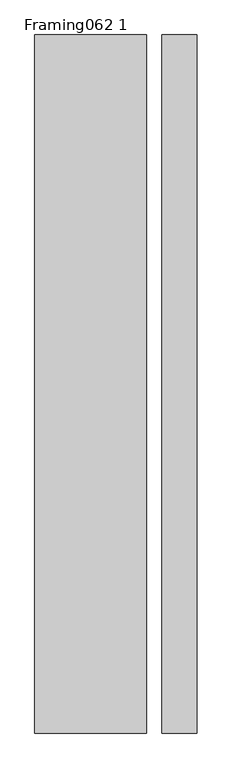
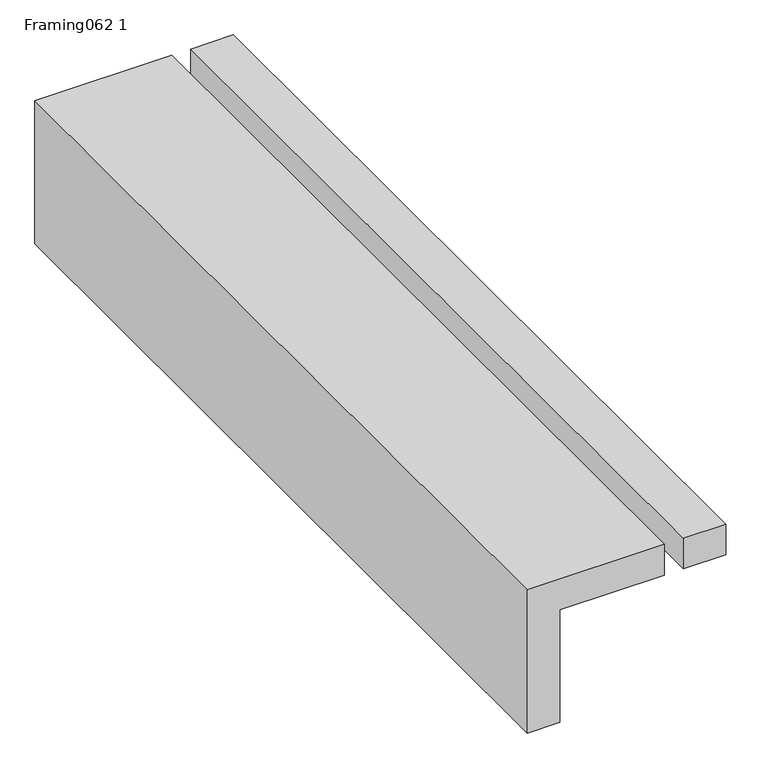
"""IFC4 building model written with IfcOpenShell, lengths in millimetres: proxy geometry, Framing062 1 : Framing062 15035."""

from ifc_helpers import new_model, si_unit, frame, origin, place, context, project, spatial, polyline, outline, extrude, source, transform, mapped, element, save


def framing062_1_cbcbbf25(model_context):
    return source(origin(), model_context, "Body", "SweptSolid", [
        extrude(outline(polyline([(42134.105552, -863.3885697), (42413.2036692, -863.3885697), (42413.2036692, -618.6019086), (42489.4036692, -618.6019086), (42489.4036692, -939.5885697), (42134.105552, -939.5885697), (42134.105552, -863.3885697)])), frame((0.0, -1052.8906574, 0.0), z_axis=(0.0, 1.0, 0.0), x_axis=(0.0, 0.0, 1.0)), (0.0, 0.0, 1.0), 2000.0),
        extrude(outline(polyline([(-474.2526923, -1052.8906574), (-574.1519086, -1052.8906574), (-574.1519086, 947.1093426), (-474.2526923, 947.1093426), (-474.2526923, -1052.8906574)])), frame((0.0, 0.0, 42413.2036692), z_axis=(0.0, 0.0, 1.0), x_axis=(1.0, 0.0, 0.0)), (0.0, 0.0, 1.0), 76.2),
    ])


if __name__ == "__main__":
    model = new_model("IFC4")
    model_context = context("Model", 3, world=origin())
    ifc_project = project(units=[si_unit("LENGTHUNIT", "METRE", prefix="MILLI")], contexts=[model_context])
    site = spatial("IfcSite", under=ifc_project)
    building = spatial("IfcBuilding", under=site)
    placement = place(None, origin())
    framing062_1_shape = framing062_1_cbcbbf25(model_context)
    element("IfcBuildingElementProxy", 1, Name="Framing062 1 : Framing062 15035", ObjectType="Framing062 1 : Framing062 15035", at=placement, inside=building, context=model_context, shape_type="MappedRepresentation", body=[
        mapped(framing062_1_shape, transform((0.0, 0.0, 0.0), x_axis=(1.0, 0.0, 0.0), y_axis=(0.0, 1.0, 0.0), z_axis=(0.0, 0.0, 1.0))),
    ])
    save(model, "model.ifc")

# Revit data of these elements
# Type "Framing062 1 : Framing062 15035"
#   NameOverride = "Framing062"
# Element 1 (IfcBuildingElementProxy, "Framing062 1 : Framing062 15035")
#   Materials on its faces: "POLYURETHANE SPRAY FOAM UNDER ROOF SUBSTRATE (SEE T-24 ENERGY REPORT FOR R-VALUE)"
# Materials
#   "POLYURETHANE SPRAY FOAM UNDER ROOF SUBSTRATE (SEE T-24 ENERGY REPORT FOR R-VALUE)": class "Unassigned", colour RGB 210 164 194, transparency 0, Cost = 0
